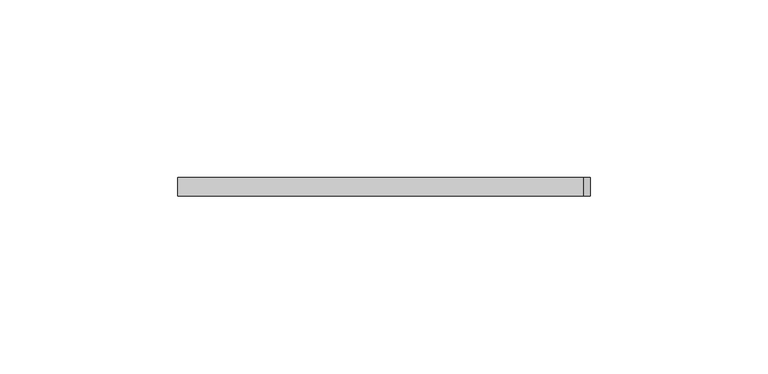
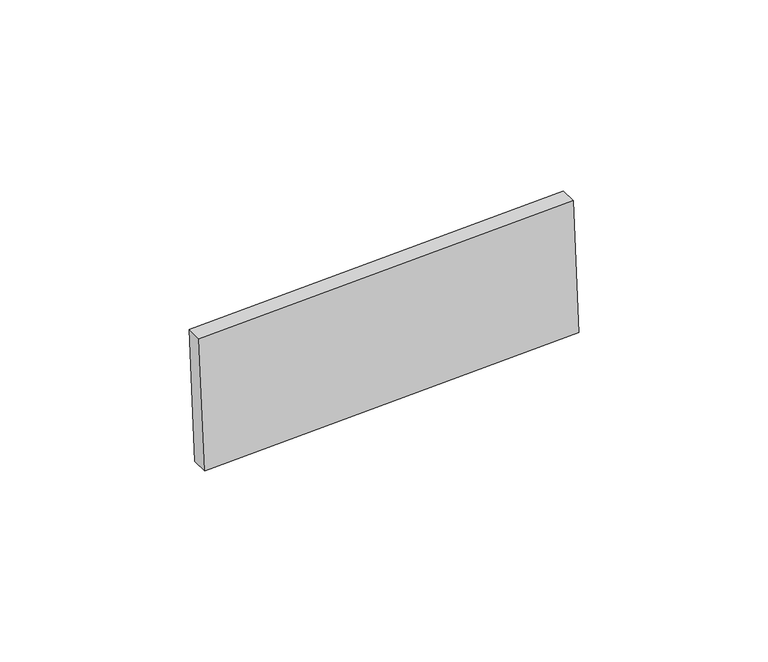
"""IFC4 building model written with IfcOpenShell, lengths in millimetres: proxy geometry, Inner panel:Inner panel:1:Inner panel:1 : Inner panel:Inner panel:300324:2:Inner panel:1:Inner panel:1 : Inner panel:Inner panel:300324:2 : Inner panel:Inner panel:1:Inner panel:1 : Inner panel:Inner panel:300324:300043:164 : Inner panel:Inner panel:1:Inner panel:1 : Inner panel:Inner panel:300324:2:Inner panel:1:Inner panel:1 : Inner panel:Inner panel:300324:2 : Inner panel:Inner panel:1:Inner panel:1 : Inner panel:Inner panel:300324:300043:308120."""

from ifc_helpers import new_model, si_unit, frame, origin, place, context, project, spatial, polyline, outline, extrude, source, transform, mapped, element, save


def generic_models_311d1274(model_context):
    return source(origin(), model_context, "Body", "SweptSolid", [
        extrude(outline(polyline([(0.0, -114.3), (0.0, 0.0), (5.213809, 0.0), (5.213809, -114.3), (0.0, -114.3)])), frame((560425.2415304, -564587.707991, 3954.8593665), z_axis=(-0.04163054471216399, 0.0, 0.9991330730923527), x_axis=(0.0, -1.0, 0.0)), (0.0, 0.0, 1.0), 43.2233908),
    ])


if __name__ == "__main__":
    model = new_model("IFC4")
    model_context = context("Model", 3, world=origin())
    ifc_project = project(units=[si_unit("LENGTHUNIT", "METRE", prefix="MILLI")], contexts=[model_context])
    site = spatial("IfcSite", under=ifc_project)
    building = spatial("IfcBuilding", under=site)
    placement = place(None, origin())
    generic_models_shape = generic_models_311d1274(model_context)
    element("IfcBuildingElementProxy", 1, Name="Inner panel:Inner panel:1:Inner panel:1 : Inner panel:Inner panel:300324:2:Inner panel:1:Inner panel:1 : Inner panel:Inner panel:300324:2 : Inner panel:Inner panel:1:Inner panel:1 : Inner panel:Inner panel:300324:300043:164 : Inner panel:Inner panel:1:Inner panel:1 : Inner panel:Inner panel:300324:2:Inner panel:1:Inner panel:1 : Inner panel:Inner panel:300324:2 : Inner panel:Inner panel:1:Inner panel:1 : Inner panel:Inner panel:300324:300043:308120", ObjectType="Inner panel:Inner panel:1:Inner panel:1 : Inner panel:Inner panel:300324:2:Inner panel:1:Inner panel:1 : Inner panel:Inner panel:300324:2 : Inner panel:Inner panel:1:Inner panel:1 : Inner panel:Inner panel:300324:300043:164 : Inner panel:Inner panel:1:Inner panel:1 : Inner panel:Inner panel:300324:2:Inner panel:1:Inner panel:1 : Inner panel:Inner panel:300324:2 : Inner panel:Inner panel:1:Inner panel:1 : Inner panel:Inner panel:300324:300043:308120", at=placement, inside=building, context=model_context, shape_type="MappedRepresentation", body=[
        mapped(generic_models_shape, transform((0.0, 0.0, 0.0), x_axis=(1.0, 0.0, 0.0), y_axis=(0.0, 1.0, 0.0), z_axis=(0.0, 0.0, 1.0))),
    ])
    save(model, "model.ifc")

# Revit data of these elements
# Type "Inner panel:Inner panel:1:Inner panel:1 : Inner panel:Inner panel:300324:2:Inner panel:1:Inner panel:1 : Inner panel:Inner panel:300324:2 : Inner panel:Inner panel:1:Inner panel:1 : Inner panel:Inner panel:300324:300043:164 : Inner panel:Inner panel:1:Inner panel:1 : Inner panel:Inner panel:300324:2:Inner panel:1:Inner panel:1 : Inner panel:Inner panel:300324:2 : Inner panel:Inner panel:1:Inner panel:1 : Inner panel:Inner panel:300324:300043:308120"
#   NameOverride = "Inner panel:Inner panel:1:Inner panel:1 : Inner panel:Inner panel:300324:2:Inner panel:1:Inner panel:1 : Inner panel:Inner panel:300324:2 : Inner panel:Inner panel:1:Inner panel:1 : Inner panel:Inner panel:300324:300043:308120"
#   ObjectTypeOverride = "Inner panel:1:Inner panel:1 : Inner panel:Inner panel:300324:2 : Inner panel:Inner panel:1:Inner panel:1 : Inner panel:Inner panel:300324:300043"
#   Reference = "Inner panel"
#   Tag = "308120"
# Element 1 (IfcBuildingElementProxy, "Inner panel:Inner panel:1:Inner panel:1 : Inner panel:Inner panel:300324:2:Inner panel:1:Inner panel:1 : Inner panel:Inner panel:300324:2 : Inner panel:Inner panel:1:Inner panel:1 : Inner panel:Inner panel:300324:300043:164 : Inner panel:Inner panel:1:Inner panel:1 : Inner panel:Inner panel:300324:2:Inner panel:1:Inner panel:1 : Inner panel:Inner panel:300324:2 : Inner panel:Inner panel:1:Inner panel:1 : Inner panel:Inner panel:300324:300043:308120")
#   Materials on its faces: "SLIDING CLIP"
# Materials
#   "SLIDING CLIP": class "Generic", colour RGB 120 120 120, transparency 0, Cost = 0
